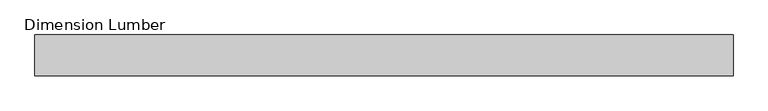
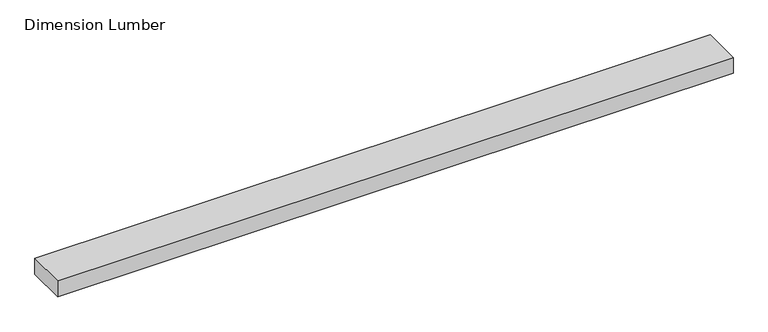
"""IFC4 building model written with IfcOpenShell, lengths in millimetres: beam geometry, Dimension Lumber : Opening Plate 2*4 Exterior."""

import ifcopenshell
import ifcopenshell.guid

model = None  # the IFC model being written
_history = None  # IfcOwnerHistory: only IFC2X3 demands one
_inside = {}  # id of a spatial element -> (the spatial element, [elements in it])
_under = {}  # id of a project, library or spatial element -> (it, [spatial elements below it])
_declared = {}  # id of a project -> (the project, [libraries it declares])
_typed = {}  # id of a type object -> (the type object, [elements of that type])
_made_of = {}  # id of a material, layer set ... -> (it, [elements and type objects made of it])


def new_model(schema):
    """Start an empty IFC model of exactly this schema.

    Asked for "IFC4X3", IfcOpenShell would pick the latest addendum, in which some entities
    have other attributes; the version numbers below select the first issue.
    IFC2X3 requires an IfcOwnerHistory on every rooted entity: one is made here for all.
    """
    global model, _history
    if schema == "IFC4X3":
        model = ifcopenshell.file(schema_version=(4, 3, 0, 0))
    else:
        model = ifcopenshell.file(schema=schema)
    _inside.clear()
    _under.clear()
    _declared.clear()
    _typed.clear()
    _made_of.clear()
    _history = None
    if model.schema == "IFC2X3":
        org = make("IfcOrganization", Name="unknown")
        user = make(
            "IfcPersonAndOrganization",
            ThePerson=make("IfcPerson", FamilyName="unknown"),
            TheOrganization=org,
        )
        app = make(
            "IfcApplication",
            ApplicationDeveloper=org,
            Version="unknown",
            ApplicationFullName="unknown",
            ApplicationIdentifier="unknown",
        )
        _history = make(
            "IfcOwnerHistory",
            OwningUser=user,
            OwningApplication=app,
            ChangeAction="ADDED",
            CreationDate=0,
        )
    return model


def make(cls, **values):
    """One entity of the class cls with the attributes given. An attribute that is None is left unset."""
    return model.create_entity(
        cls, **{name: value for name, value in values.items() if value is not None}
    )


def rooted(cls, **values):
    """An entity with a GlobalId (a new one), such as an element, a storey or a relation."""
    return make(cls, GlobalId=ifcopenshell.guid.new(), OwnerHistory=_history, **values)


def si_unit(unit_type, name, prefix=None):
    """IfcSIUnit, for example si_unit("LENGTHUNIT", "METRE", prefix="MILLI")."""
    return make("IfcSIUnit", UnitType=unit_type, Prefix=prefix, Name=name)


def assignment(units):
    """IfcUnitAssignment: the units of a project."""
    return None if units is None else make("IfcUnitAssignment", Units=units)


def point(xyz):
    """IfcCartesianPoint."""
    return None if xyz is None else make("IfcCartesianPoint", Coordinates=xyz)


def direction(xyz):
    """IfcDirection."""
    return None if xyz is None else make("IfcDirection", DirectionRatios=xyz)


def frame(location, z_axis=None, x_axis=None):
    """IfcAxis2Placement3D, a coordinate frame: its origin and axes. An axis left out is left unset."""
    return make(
        "IfcAxis2Placement3D",
        Location=point(location),
        Axis=direction(z_axis),
        RefDirection=direction(x_axis),
    )


def origin():
    """The frame at (0, 0, 0) with its axes left unset."""
    return frame((0.0, 0.0, 0.0))


def place(relative_to, where):
    """IfcLocalPlacement: puts the frame where relative to a parent placement (None: the world)."""
    return make(
        "IfcLocalPlacement", PlacementRelTo=relative_to, RelativePlacement=where
    )


def context(
    kind, dimensions, precision=None, world=None, true_north=None, identifier=None
):
    """IfcGeometricRepresentationContext, for example the 3D "Model" context."""
    return make(
        "IfcGeometricRepresentationContext",
        ContextIdentifier=identifier,
        ContextType=kind,
        CoordinateSpaceDimension=dimensions,
        Precision=precision,
        WorldCoordinateSystem=world,
        TrueNorth=true_north,
    )


def project(units=None, contexts=None):
    """IfcProject with its units and contexts."""
    return rooted(
        "IfcProject",
        Name="project",
        RepresentationContexts=contexts,
        UnitsInContext=assignment(units),
    )


def spatial(cls, under=None, at=None, **own):
    """A site, building, storey or space (cls), placed at a placement, below another one or the project."""
    s = rooted(cls, ObjectPlacement=at, **own)
    if under is not None:
        _under.setdefault(under.id(), (under, []))[1].append(s)
    return s


def polyline(points):
    """IfcPolyline through the points."""
    return make("IfcPolyline", Points=[point(p) for p in points])


def outline(outer, holes=None, kind="AREA"):
    """IfcArbitraryClosedProfileDef: a profile drawn as a closed curve; with holes, ...WithVoids."""
    if holes is None:
        return make("IfcArbitraryClosedProfileDef", ProfileType=kind, OuterCurve=outer)
    return make(
        "IfcArbitraryProfileDefWithVoids",
        ProfileType=kind,
        OuterCurve=outer,
        InnerCurves=holes,
    )


def extrude(swept, where, along, depth):
    """IfcExtrudedAreaSolid: the profile swept, set in the frame where, extruded along a direction by depth."""
    return make(
        "IfcExtrudedAreaSolid",
        SweptArea=swept,
        Position=where,
        ExtrudedDirection=direction(along),
        Depth=depth,
    )


def shape(context_of_items, identifier, shape_type, items):
    """IfcShapeRepresentation: the items that make up one representation, for example the "Body"."""
    return make(
        "IfcShapeRepresentation",
        ContextOfItems=context_of_items,
        RepresentationIdentifier=identifier,
        RepresentationType=shape_type,
        Items=items,
    )


def source(mapping_origin, context_of_items, identifier, shape_type, items):
    """IfcRepresentationMap: a shape defined once, which mapped items show again and again."""
    return make(
        "IfcRepresentationMap",
        MappingOrigin=mapping_origin,
        MappedRepresentation=shape(context_of_items, identifier, shape_type, items),
    )


def transform(
    local_origin,
    x_axis=None,
    y_axis=None,
    z_axis=None,
    scale=None,
    scale2=None,
    scale3=None,
    uniform=True,
):
    """IfcCartesianTransformationOperator3D, or its non-uniform kind. x_axis, y_axis, z_axis: its Axis1, 2, 3."""
    if uniform:
        return make(
            "IfcCartesianTransformationOperator3D",
            Axis1=direction(x_axis),
            Axis2=direction(y_axis),
            LocalOrigin=point(local_origin),
            Scale=scale,
            Axis3=direction(z_axis),
        )
    return make(
        "IfcCartesianTransformationOperator3DnonUniform",
        Axis1=direction(x_axis),
        Axis2=direction(y_axis),
        LocalOrigin=point(local_origin),
        Scale=scale,
        Axis3=direction(z_axis),
        Scale2=scale2,
        Scale3=scale3,
    )


def mapped(mapping_source, mapping_target):
    """IfcMappedItem: shows the shape of a source again, moved by a transform."""
    return make(
        "IfcMappedItem", MappingSource=mapping_source, MappingTarget=mapping_target
    )


def made_of(thing, what):
    """Note that an element or type object is made of a material, layer set ...; save() writes the relation."""
    if what is not None:
        _made_of.setdefault(what.id(), (what, []))[1].append(thing)
    return thing


def element(
    cls,
    number,
    at=None,
    inside=None,
    cuts=None,
    type_object=None,
    material=None,
    context=None,
    identifier="Body",
    shape_type=None,
    held_by="IfcProductDefinitionShape",
    body=None,
    shapes=None,
    **own,
):
    """One element of the class cls, such as IfcWall. Its Tag is "e" and its number.

    at: its placement. inside: the storey or other place that contains it. cuts: it is an
    opening in that element (IfcRelVoidsElement). A single representation is given by context,
    identifier, shape_type and body (its items); several are given by shapes. held_by: the class
    of the entity that holds the representations. save() writes the other relations.
    """
    e = rooted(cls, Tag="e%d" % number, ObjectPlacement=at, **own)
    if body is not None:
        shapes = [shape(context, identifier, shape_type, body)]
    if shapes is not None:
        e.Representation = make(held_by, Representations=shapes)
    if inside is not None:
        _inside.setdefault(inside.id(), (inside, []))[1].append(e)
    if cuts is not None:
        rooted(
            "IfcRelVoidsElement", RelatingBuildingElement=cuts, RelatedOpeningElement=e
        )
    if type_object is not None:
        _typed.setdefault(type_object.id(), (type_object, []))[1].append(e)
    return made_of(e, material)


def aggregate(whole, parts):
    """IfcRelAggregates: a whole, such as a stair, and the parts it consists of."""
    return rooted("IfcRelAggregates", RelatingObject=whole, RelatedObjects=parts)


def save(model, path):
    """Write the relations noted so far, then the file.

    IfcRelAggregates (storeys below a building ...), IfcRelContainedInSpatialStructure (elements
    in a storey), IfcRelDefinesByType, IfcRelAssociatesMaterial and IfcRelDeclares: one each for
    every whole, place, type object, material and project.
    """
    for whole, parts in _under.values():
        aggregate(whole, parts)
    for where, things in _inside.values():
        rooted(
            "IfcRelContainedInSpatialStructure",
            RelatedElements=things,
            RelatingStructure=where,
        )
    for kind, things in _typed.values():
        rooted("IfcRelDefinesByType", RelatedObjects=things, RelatingType=kind)
    for what, things in _made_of.values():
        rooted("IfcRelAssociatesMaterial", RelatedObjects=things, RelatingMaterial=what)
    for by, libraries in _declared.values():
        rooted("IfcRelDeclares", RelatingContext=by, RelatedDefinitions=libraries)
    model.write(path)


def dimension_lumber_9d951cb9(model_context):
    return source(origin(), model_context, "Body", "SweptSolid", [
        extrude(outline(polyline([(752.4750003, 44.45), (752.4750003, -44.45), (-771.5249997, -44.45), (-771.5249997, 44.45), (752.4750003, 44.45)])), frame((0.0, 0.0, -19.05), z_axis=(0.0, 0.0, 1.0), x_axis=(1.0, 0.0, 0.0)), (0.0, 0.0, 1.0), 38.1),
    ])


if __name__ == "__main__":
    model = new_model("IFC4")
    model_context = context("Model", 3, world=origin())
    ifc_project = project(units=[si_unit("LENGTHUNIT", "METRE", prefix="MILLI")], contexts=[model_context])
    site = spatial("IfcSite", under=ifc_project)
    building = spatial("IfcBuilding", under=site)
    placement = place(None, origin())
    dimension_lumber_shape = dimension_lumber_9d951cb9(model_context)
    element("IfcBeam", 1, ObjectType="Dimension Lumber : Opening Plate 2*4 Exterior", at=placement, inside=building, context=model_context, shape_type="MappedRepresentation", body=[
        mapped(dimension_lumber_shape, transform((0.0, 0.0, 0.0), x_axis=(1.0, 0.0, 0.0), y_axis=(0.0, 1.0, 0.0), z_axis=(0.0, 0.0, 1.0))),
    ])
    save(model, "model.ifc")

# Revit data of these elements
# Type "Dimension Lumber : Opening Plate 2*4 Exterior"
#   Assembly Code = "B10"
#   A = 0.0364583 SF
#   Length [instance default] = 5' - 0"
#   b = 0' - 3 1/2"
#   d = 0' - 1 1/2"
#   Structural Material [instance default] = Softwood, Lumber
# Element 1 (IfcBeam, "Dimension Lumber : Opening Plate 2*4 Exterior")
#   Structural Material = Douglas Fir #2
#   Materials on its faces: "Douglas Fir #2"
# Materials
#   "Softwood, Lumber": class "Wood", colour RGB 223 192 134, transparency 0, Description = "Pinus Echinata", Cost = 0
#   "Douglas Fir #2": class "Wood", colour RGB 223 192 134, transparency 0, Description = "Pinus Echinata", Cost = 0
